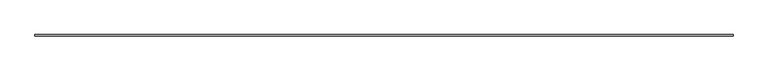
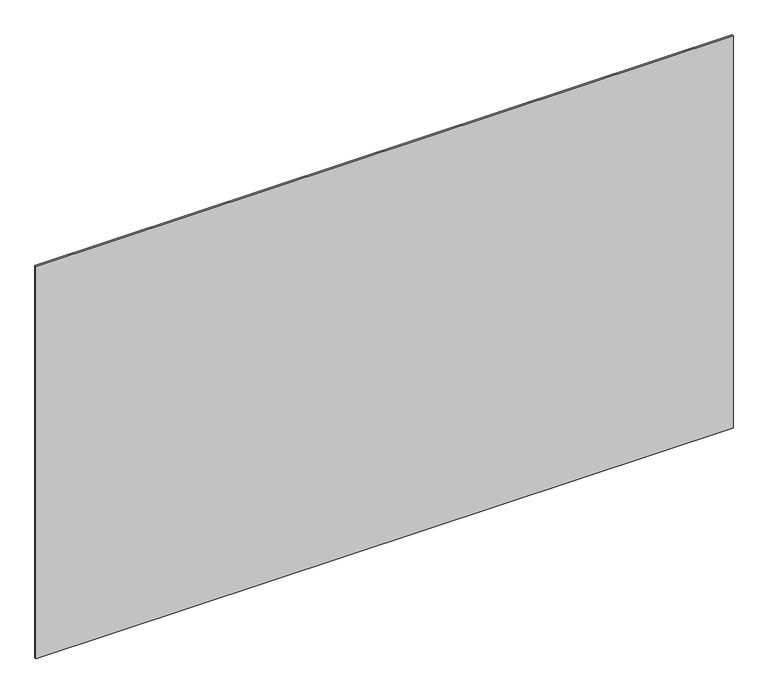
"""IFC4 building model written with IfcOpenShell, lengths in millimetres: plate geometry, 系统嵌板 : 玻璃."""

from ifc_helpers import new_model, si_unit, origin, origin_with_axes, place, context, project, spatial, polyline, outline, extrude, source, transform, mapped, element, save


def plate_433a51a3(model_context):
    return source(origin(), model_context, "Body", "SweptSolid", [
        extrude(outline(polyline([(6050.0, -12.5), (-6050.0, -12.5), (-6050.0, 12.5), (6050.0, 12.5), (6050.0, -12.5)])), origin_with_axes(), (0.0, 0.0, 1.0), 7200.0),
    ])


if __name__ == "__main__":
    model = new_model("IFC4")
    model_context = context("Model", 3, world=origin())
    ifc_project = project(units=[si_unit("LENGTHUNIT", "METRE", prefix="MILLI")], contexts=[model_context])
    site = spatial("IfcSite", under=ifc_project)
    building = spatial("IfcBuilding", under=site)
    placement = place(None, origin())
    plate_shape = plate_433a51a3(model_context)
    element("IfcPlate", 1, ObjectType="系统嵌板 : 玻璃", at=placement, inside=building, context=model_context, shape_type="MappedRepresentation", body=[
        mapped(plate_shape, transform((0.0, 0.0, 0.0), x_axis=(1.0, 0.0, 0.0), y_axis=(0.0, 1.0, 0.0), z_axis=(0.0, 0.0, 1.0))),
    ])
    save(model, "model.ifc")

# Revit data of these elements
# Type "系统嵌板 : 玻璃"
#   Construction Type Id = "GSP4R"
#   Analytic Construction = "1/8 英寸 Pilkington 单层玻璃"
#   Visual Light Transmittance = 0.9
#   Solar Heat Gain Coefficient = 0.86
#   Heat Transfer Coefficient (U) = 6.7069 W/(m²·K)
# Element 1 (IfcPlate, "系统嵌板 : 玻璃")
#   Materials on its faces: "玻璃"
# Materials
#   "玻璃": class "玻璃", colour RGB 0 128 192, transparency 0.9, Description = "钠钙玻璃", Cost = 0
